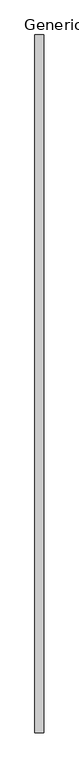
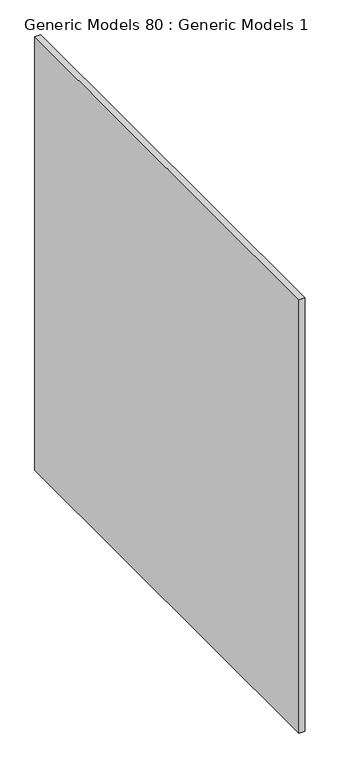
"""IFC4 building model written with IfcOpenShell, lengths in millimetres: proxy geometry, Generic Models 80 : Generic Models 1."""

from ifc_helpers import new_model, si_unit, frame, origin, place, context, project, spatial, polyline, outline, extrude, source, transform, mapped, element, save


def generic_models_80_generic_models_1_dd39fccb(model_context):
    return source(origin(), model_context, "Body", "SweptSolid", [
        extrude(outline(polyline([(46951.7485531, 1219.2), (46951.7485531, 0.0), (46935.8735531, 0.0), (46935.8735531, 1219.2), (46951.7485531, 1219.2)])), frame((0.0, 0.0, -219.626067), z_axis=(0.0, 0.0, 1.0), x_axis=(1.0, 0.0, 0.0)), (0.0, 0.0, 1.0), 1219.2),
    ])


if __name__ == "__main__":
    model = new_model("IFC4")
    model_context = context("Model", 3, world=origin())
    ifc_project = project(units=[si_unit("LENGTHUNIT", "METRE", prefix="MILLI")], contexts=[model_context])
    site = spatial("IfcSite", under=ifc_project)
    building = spatial("IfcBuilding", under=site)
    placement = place(None, origin())
    generic_models_80_generic_models_1_shape = generic_models_80_generic_models_1_dd39fccb(model_context)
    element("IfcBuildingElementProxy", 1, Name="Generic Models 80 : Generic Models 1", ObjectType="Generic Models 80 : Generic Models 1", at=placement, inside=building, context=model_context, shape_type="MappedRepresentation", body=[
        mapped(generic_models_80_generic_models_1_shape, transform((0.0, 0.0, 0.0), x_axis=(1.0, 0.0, 0.0), y_axis=(0.0, 1.0, 0.0), z_axis=(0.0, 0.0, 1.0))),
    ])
    save(model, "model.ifc")

# Revit data of these elements
# Element 1 (IfcBuildingElementProxy, "Generic Models 80 : Generic Models 1")
#   Materials on its faces: "5/8\" GYP. BD"
# Materials
#   "5/8\" GYP. BD": class "Generic", colour RGB 255 255 255, transparency 0, Description = "Gypsum Wall Board", Cost = 0
